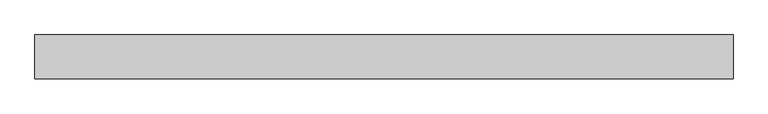
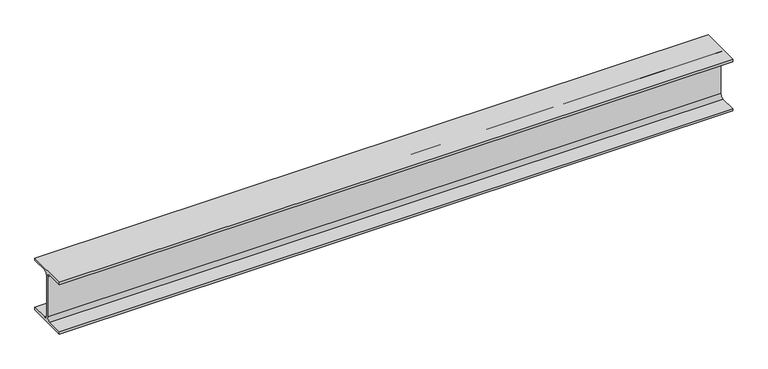
"""IFC4 building model written with IfcOpenShell, lengths in millimetres: beam geometry, 0912_Steel Framing_H-KSD3502 : H_SB_ASB_H-194x150x6x9."""

import ifcopenshell
import ifcopenshell.guid

model = None  # the IFC model being written
_history = None  # IfcOwnerHistory: only IFC2X3 demands one
_inside = {}  # id of a spatial element -> (the spatial element, [elements in it])
_under = {}  # id of a project, library or spatial element -> (it, [spatial elements below it])
_declared = {}  # id of a project -> (the project, [libraries it declares])
_typed = {}  # id of a type object -> (the type object, [elements of that type])
_made_of = {}  # id of a material, layer set ... -> (it, [elements and type objects made of it])


def new_model(schema):
    """Start an empty IFC model of exactly this schema.

    Asked for "IFC4X3", IfcOpenShell would pick the latest addendum, in which some entities
    have other attributes; the version numbers below select the first issue.
    IFC2X3 requires an IfcOwnerHistory on every rooted entity: one is made here for all.
    """
    global model, _history
    if schema == "IFC4X3":
        model = ifcopenshell.file(schema_version=(4, 3, 0, 0))
    else:
        model = ifcopenshell.file(schema=schema)
    _inside.clear()
    _under.clear()
    _declared.clear()
    _typed.clear()
    _made_of.clear()
    _history = None
    if model.schema == "IFC2X3":
        org = make("IfcOrganization", Name="unknown")
        user = make(
            "IfcPersonAndOrganization",
            ThePerson=make("IfcPerson", FamilyName="unknown"),
            TheOrganization=org,
        )
        app = make(
            "IfcApplication",
            ApplicationDeveloper=org,
            Version="unknown",
            ApplicationFullName="unknown",
            ApplicationIdentifier="unknown",
        )
        _history = make(
            "IfcOwnerHistory",
            OwningUser=user,
            OwningApplication=app,
            ChangeAction="ADDED",
            CreationDate=0,
        )
    return model


def make(cls, **values):
    """One entity of the class cls with the attributes given. An attribute that is None is left unset."""
    return model.create_entity(
        cls, **{name: value for name, value in values.items() if value is not None}
    )


def rooted(cls, **values):
    """An entity with a GlobalId (a new one), such as an element, a storey or a relation."""
    return make(cls, GlobalId=ifcopenshell.guid.new(), OwnerHistory=_history, **values)


def si_unit(unit_type, name, prefix=None):
    """IfcSIUnit, for example si_unit("LENGTHUNIT", "METRE", prefix="MILLI")."""
    return make("IfcSIUnit", UnitType=unit_type, Prefix=prefix, Name=name)


def assignment(units):
    """IfcUnitAssignment: the units of a project."""
    return None if units is None else make("IfcUnitAssignment", Units=units)


def point(xyz):
    """IfcCartesianPoint."""
    return None if xyz is None else make("IfcCartesianPoint", Coordinates=xyz)


def direction(xyz):
    """IfcDirection."""
    return None if xyz is None else make("IfcDirection", DirectionRatios=xyz)


def frame(location, z_axis=None, x_axis=None):
    """IfcAxis2Placement3D, a coordinate frame: its origin and axes. An axis left out is left unset."""
    return make(
        "IfcAxis2Placement3D",
        Location=point(location),
        Axis=direction(z_axis),
        RefDirection=direction(x_axis),
    )


def frame_2d(location, x_axis=None):
    """IfcAxis2Placement2D, a coordinate frame in the plane: its origin and x axis."""
    return make(
        "IfcAxis2Placement2D", Location=point(location), RefDirection=direction(x_axis)
    )


def origin():
    """The frame at (0, 0, 0) with its axes left unset."""
    return frame((0.0, 0.0, 0.0))


def place(relative_to, where):
    """IfcLocalPlacement: puts the frame where relative to a parent placement (None: the world)."""
    return make(
        "IfcLocalPlacement", PlacementRelTo=relative_to, RelativePlacement=where
    )


def context(
    kind, dimensions, precision=None, world=None, true_north=None, identifier=None
):
    """IfcGeometricRepresentationContext, for example the 3D "Model" context."""
    return make(
        "IfcGeometricRepresentationContext",
        ContextIdentifier=identifier,
        ContextType=kind,
        CoordinateSpaceDimension=dimensions,
        Precision=precision,
        WorldCoordinateSystem=world,
        TrueNorth=true_north,
    )


def project(units=None, contexts=None):
    """IfcProject with its units and contexts."""
    return rooted(
        "IfcProject",
        Name="project",
        RepresentationContexts=contexts,
        UnitsInContext=assignment(units),
    )


def spatial(cls, under=None, at=None, **own):
    """A site, building, storey or space (cls), placed at a placement, below another one or the project."""
    s = rooted(cls, ObjectPlacement=at, **own)
    if under is not None:
        _under.setdefault(under.id(), (under, []))[1].append(s)
    return s


def polyline(points):
    """IfcPolyline through the points."""
    return make("IfcPolyline", Points=[point(p) for p in points])


def circle_curve(where, radius):
    """IfcCircle in the frame where."""
    return make("IfcCircle", Position=where, Radius=radius)


def trimmed(basis, trim1, trim2, sense, master):
    """IfcTrimmedCurve: the piece of a basis curve between two trims."""
    return make(
        "IfcTrimmedCurve",
        BasisCurve=basis,
        Trim1=trim1,
        Trim2=trim2,
        SenseAgreement=sense,
        MasterRepresentation=master,
    )


def segment(curve, same_sense, transition):
    """IfcCompositeCurveSegment."""
    return make(
        "IfcCompositeCurveSegment",
        Transition=transition,
        SameSense=same_sense,
        ParentCurve=curve,
    )


def composite_curve(segments, self_intersect=None):
    """IfcCompositeCurve: segments joined end to end."""
    return make("IfcCompositeCurve", Segments=segments, SelfIntersect=self_intersect)


def outline(outer, holes=None, kind="AREA"):
    """IfcArbitraryClosedProfileDef: a profile drawn as a closed curve; with holes, ...WithVoids."""
    if holes is None:
        return make("IfcArbitraryClosedProfileDef", ProfileType=kind, OuterCurve=outer)
    return make(
        "IfcArbitraryProfileDefWithVoids",
        ProfileType=kind,
        OuterCurve=outer,
        InnerCurves=holes,
    )


def extrude(swept, where, along, depth):
    """IfcExtrudedAreaSolid: the profile swept, set in the frame where, extruded along a direction by depth."""
    return make(
        "IfcExtrudedAreaSolid",
        SweptArea=swept,
        Position=where,
        ExtrudedDirection=direction(along),
        Depth=depth,
    )


def shape(context_of_items, identifier, shape_type, items):
    """IfcShapeRepresentation: the items that make up one representation, for example the "Body"."""
    return make(
        "IfcShapeRepresentation",
        ContextOfItems=context_of_items,
        RepresentationIdentifier=identifier,
        RepresentationType=shape_type,
        Items=items,
    )


def source(mapping_origin, context_of_items, identifier, shape_type, items):
    """IfcRepresentationMap: a shape defined once, which mapped items show again and again."""
    return make(
        "IfcRepresentationMap",
        MappingOrigin=mapping_origin,
        MappedRepresentation=shape(context_of_items, identifier, shape_type, items),
    )


def transform(
    local_origin,
    x_axis=None,
    y_axis=None,
    z_axis=None,
    scale=None,
    scale2=None,
    scale3=None,
    uniform=True,
):
    """IfcCartesianTransformationOperator3D, or its non-uniform kind. x_axis, y_axis, z_axis: its Axis1, 2, 3."""
    if uniform:
        return make(
            "IfcCartesianTransformationOperator3D",
            Axis1=direction(x_axis),
            Axis2=direction(y_axis),
            LocalOrigin=point(local_origin),
            Scale=scale,
            Axis3=direction(z_axis),
        )
    return make(
        "IfcCartesianTransformationOperator3DnonUniform",
        Axis1=direction(x_axis),
        Axis2=direction(y_axis),
        LocalOrigin=point(local_origin),
        Scale=scale,
        Axis3=direction(z_axis),
        Scale2=scale2,
        Scale3=scale3,
    )


def mapped(mapping_source, mapping_target):
    """IfcMappedItem: shows the shape of a source again, moved by a transform."""
    return make(
        "IfcMappedItem", MappingSource=mapping_source, MappingTarget=mapping_target
    )


def made_of(thing, what):
    """Note that an element or type object is made of a material, layer set ...; save() writes the relation."""
    if what is not None:
        _made_of.setdefault(what.id(), (what, []))[1].append(thing)
    return thing


def element(
    cls,
    number,
    at=None,
    inside=None,
    cuts=None,
    type_object=None,
    material=None,
    context=None,
    identifier="Body",
    shape_type=None,
    held_by="IfcProductDefinitionShape",
    body=None,
    shapes=None,
    **own,
):
    """One element of the class cls, such as IfcWall. Its Tag is "e" and its number.

    at: its placement. inside: the storey or other place that contains it. cuts: it is an
    opening in that element (IfcRelVoidsElement). A single representation is given by context,
    identifier, shape_type and body (its items); several are given by shapes. held_by: the class
    of the entity that holds the representations. save() writes the other relations.
    """
    e = rooted(cls, Tag="e%d" % number, ObjectPlacement=at, **own)
    if body is not None:
        shapes = [shape(context, identifier, shape_type, body)]
    if shapes is not None:
        e.Representation = make(held_by, Representations=shapes)
    if inside is not None:
        _inside.setdefault(inside.id(), (inside, []))[1].append(e)
    if cuts is not None:
        rooted(
            "IfcRelVoidsElement", RelatingBuildingElement=cuts, RelatedOpeningElement=e
        )
    if type_object is not None:
        _typed.setdefault(type_object.id(), (type_object, []))[1].append(e)
    return made_of(e, material)


def aggregate(whole, parts):
    """IfcRelAggregates: a whole, such as a stair, and the parts it consists of."""
    return rooted("IfcRelAggregates", RelatingObject=whole, RelatedObjects=parts)


def save(model, path):
    """Write the relations noted so far, then the file.

    IfcRelAggregates (storeys below a building ...), IfcRelContainedInSpatialStructure (elements
    in a storey), IfcRelDefinesByType, IfcRelAssociatesMaterial and IfcRelDeclares: one each for
    every whole, place, type object, material and project.
    """
    for whole, parts in _under.values():
        aggregate(whole, parts)
    for where, things in _inside.values():
        rooted(
            "IfcRelContainedInSpatialStructure",
            RelatedElements=things,
            RelatingStructure=where,
        )
    for kind, things in _typed.values():
        rooted("IfcRelDefinesByType", RelatedObjects=things, RelatingType=kind)
    for what, things in _made_of.values():
        rooted("IfcRelAssociatesMaterial", RelatedObjects=things, RelatingMaterial=what)
    for by, libraries in _declared.values():
        rooted("IfcRelDeclares", RelatingContext=by, RelatedDefinitions=libraries)
    model.write(path)


def beam_830b10b4(model_context):
    return source(origin(), model_context, "Body", "SweptSolid", [
        extrude(outline(composite_curve([segment(polyline([(75.0, -88.0), (75.0, -97.0), (-75.0, -97.0), (-75.0, -88.0), (-16.0, -88.0)]), True, "CONTINUOUS"), segment(trimmed(circle_curve(frame_2d((-16.0, -75.0)), 13.0), [point((-16.0, -88.0))], [point((-3.0, -75.0))], True, "CARTESIAN"), True, "CONTINUOUS"), segment(polyline([(-3.0, -75.0), (-3.0, 75.0)]), True, "CONTINUOUS"), segment(trimmed(circle_curve(frame_2d((-16.0, 75.0)), 13.0), [point((-3.0, 75.0))], [point((-16.0, 88.0))], True, "CARTESIAN"), True, "CONTINUOUS"), segment(polyline([(-16.0, 88.0), (-75.0, 88.0), (-75.0, 97.0), (75.0, 97.0), (75.0, 88.0), (16.0, 88.0)]), True, "CONTINUOUS"), segment(trimmed(circle_curve(frame_2d((16.0, 75.0)), 13.0), [point((16.0, 88.0))], [point((3.0, 75.0))], True, "CARTESIAN"), True, "CONTINUOUS"), segment(polyline([(3.0, 75.0), (3.0, -75.0)]), True, "CONTINUOUS"), segment(trimmed(circle_curve(frame_2d((16.0, -75.0)), 13.0), [point((3.0, -75.0))], [point((16.0, -88.0))], True, "CARTESIAN"), True, "CONTINUOUS"), segment(polyline([(16.0, -88.0), (75.0, -88.0)]), True, "CONTINUOUS")], self_intersect=False)), frame((-1520.0832263, 0.0, 0.0), z_axis=(1.0, 0.0, 0.0), x_axis=(0.0, 1.0, 0.0)), (0.0, 0.0, 1.0), 2387.3),
    ])


if __name__ == "__main__":
    model = new_model("IFC4")
    model_context = context("Model", 3, world=origin())
    ifc_project = project(units=[si_unit("LENGTHUNIT", "METRE", prefix="MILLI")], contexts=[model_context])
    site = spatial("IfcSite", under=ifc_project)
    building = spatial("IfcBuilding", under=site)
    placement = place(None, origin())
    beam_shape = beam_830b10b4(model_context)
    element("IfcBeam", 1, ObjectType="0912_Steel Framing_H-KSD3502 : H_SB_ASB_H-194x150x6x9", at=placement, inside=building, context=model_context, shape_type="MappedRepresentation", body=[
        mapped(beam_shape, transform((0.0, 0.0, 0.0), x_axis=(1.0, 0.0, 0.0), y_axis=(0.0, 1.0, 0.0), z_axis=(0.0, 0.0, 1.0))),
    ])
    save(model, "model.ifc")

# Revit data of these elements
# Type "0912_Steel Framing_H-KSD3502 : H_SB_ASB_H-194x150x6x9"
#   H_WM Code_1 = "S01AA002-00001 | Main Steel Structure Fabrication Work | Shelter/Building | Medium Steel - Standard (90KG/M>Weight≥30KG/M) | Material: (   )"
#   H_WM Code_2 = "S03AA028-00001 | Main Steel Structure Erection Work | Shelter/Building | Medium Steel (90KG/M>Weight≥30KG/M) | Material: (   )"
#   H_WM Code_3 = "S01AA010-00001 | Main Steel Structure Fabrication Work | Shelter/Building | Steel Painting/Coating | for Non-Fireproofed Steel Surface, Surface Preparation, Primer, Second & Final Coat | Material: (   )"
#   H_Q'ty Cal Type Tag = "SB-Q2"
#   Width = 15.0 cm
#   Web Thickness = 0.6 cm
#   Web Fillet = 1.3 cm
#   Warping Constant = 43316.0 cm⁶
#   W = 0
#   Torsional Moment of Inertia = 8.622 cm⁴
#   Section Area = 39.01 cm²
#   Plastic Modulus weak axis = 104.0 cm³
#   Plastic Modulus strong axis = 309.0 cm³
#   Perimeter = 0.95 m²/m
#   Nominal Weight = 30.60 kgf/m
#   Moment of Inertia weak axis = 507.00 cm⁴
#   Moment of Inertia strong axis = 2690.00 cm⁴
#   Height = 19.4 cm
#   Flange Thickness = 0.9 cm
#   Elastic Modulus weak axis = 67.6 cm³
#   Elastic Modulus strong axis = 277.0 cm³
#   Centroid Vertical = 9.7 cm
#   Centroid Horizontal = 7.5 cm
#   Ix = 26900000
#   Length [instance default] = 1.5240 m
#   Zx = 309000
#   b = 0.1500 m
#   h = 0.1940 m
#   r = 0.0130 m
#   s = 0.0060 m
#   t = 0.0090 m
#   A = 0.003901 m²
#   Structural Material [instance default] = Steel, 45-345
#   Assembly Code = ""
# Element 1 (IfcBeam, "0912_Steel Framing_H-KSD3502 : H_SB_ASB_H-194x150x6x9")
#   Structural Material = none
# Materials
#   "Steel, 45-345": class "Metal", colour RGB 189 187 185, transparency 0, Description = "Steel 345 MPa", Cost = 0
